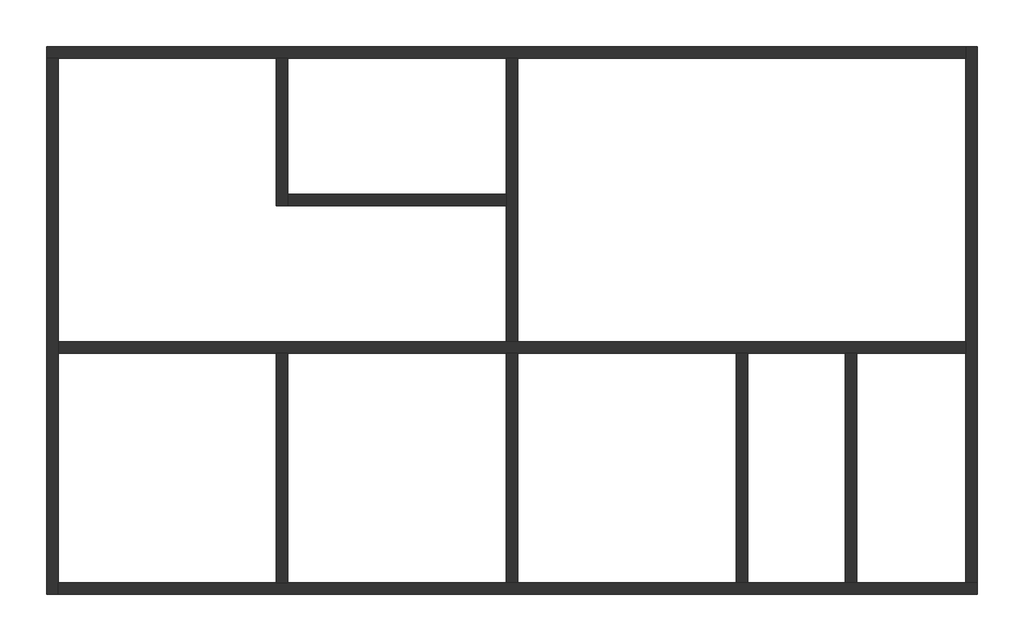
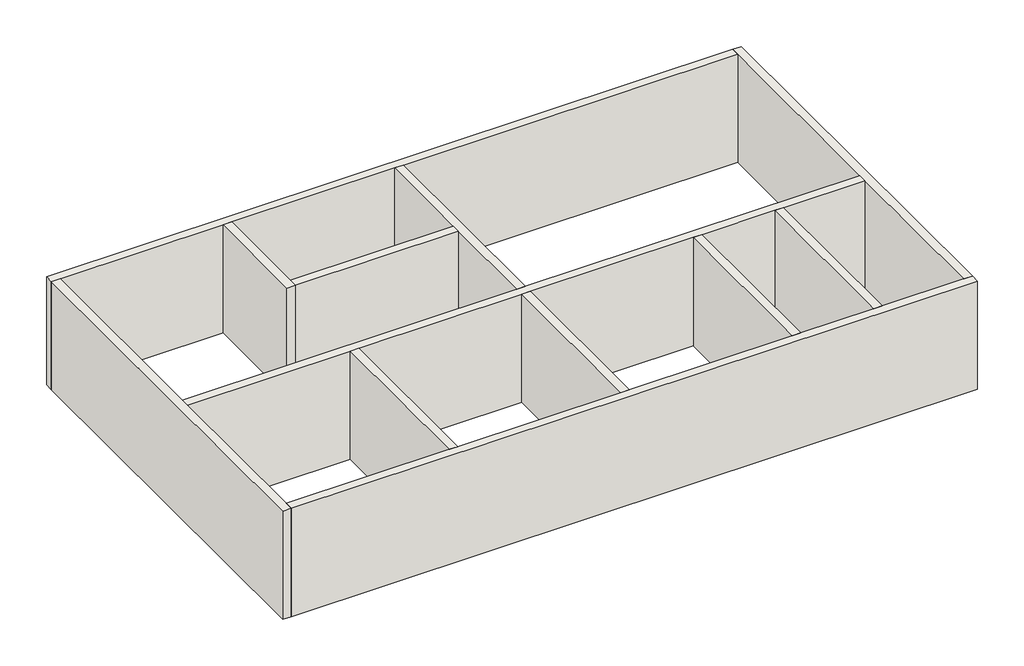
# One storey: 12 walls.
"""IFC4 building model written with IfcOpenShell, lengths in millimetres."""

from ifc_helpers import new_model, si_unit, frame, origin, place, context, project, spatial, polyline, outline, extrude, faceted_brep, element, save

model = new_model("IFC4")

# Units and contexts
model_context = context("Model", 3, world=origin())
ifc_project = project(units=[si_unit("LENGTHUNIT", "METRE", prefix="MILLI")], contexts=[model_context])

# Site, building, storey
site = spatial("IfcSite", under=ifc_project)
building = spatial("IfcBuilding", under=site)
storey = spatial("IfcBuildingStorey", under=building, Name="2nd FL GL+6,200", Elevation=6000.0)

# Walls
placement = place(None, origin())
element("IfcWall", 1, ObjectType="일반 - 300mm", at=placement, inside=storey, context=model_context, shape_type="Brep", body=[
    faceted_brep([(-18845.7273237, 9285.9763125, 6000.0), (-18545.7273237, 9285.9763125, 6000.0), (-12845.7273237, 9285.9763125, 6000.0), (-12545.7273237, 9285.9763125, 6000.0), (-6845.7273237, 9285.9763125, 6000.0), (-6545.7273237, 9285.9763125, 6000.0), (5154.2726763, 9285.9763125, 6000.0), (5154.2726763, 9285.9763125, 10000.0), (-6545.7273237, 9285.9763125, 10000.0), (-6845.7273237, 9285.9763125, 10000.0), (-12545.7273237, 9285.9763125, 10000.0), (-12845.7273237, 9285.9763125, 10000.0), (-18545.7273237, 9285.9763125, 10000.0), (-18845.7273237, 9285.9763125, 10000.0), (-18845.7273237, 9585.9763125, 6000.0), (-18845.7273237, 9585.9763125, 10000.0), (5154.2726763, 9585.9763125, 10000.0), (5154.2726763, 9585.9763125, 6000.0)], [[[0, 1, 2, 3, 4, 5, 6, 7, 8, 9, 10, 11, 12, 13]], [[14, 15, 16, 17]], [[6, 5, 4, 3, 2, 1, 0, 14, 17]], [[13, 12, 11, 10, 9, 8, 7, 16, 15]], [[0, 13, 15, 14]], [[7, 6, 17, 16]]]),
])
element("IfcWall", 2, ObjectType="일반 - 300mm", at=placement, inside=storey, context=model_context, shape_type="Brep", body=[
    faceted_brep([(-18545.7273237, -4714.0236875, 6000.0), (-18545.7273237, -4414.0236875, 6000.0), (-18545.7273237, 1585.9763125, 6000.0), (-18545.7273237, 1885.9763125, 6000.0), (-18545.7273237, 9285.9763125, 6000.0), (-18545.7273237, 9285.9763125, 10000.0), (-18545.7273237, 1885.9763125, 10000.0), (-18545.7273237, 1585.9763125, 10000.0), (-18545.7273237, -4414.0236875, 10000.0), (-18545.7273237, -4714.0236875, 10000.0), (-18845.7273237, -4714.0236875, 6000.0), (-18845.7273237, -4714.0236875, 10000.0), (-18845.7273237, 9285.9763125, 10000.0), (-18845.7273237, 9285.9763125, 6000.0)], [[[0, 1, 2, 3, 4, 5, 6, 7, 8, 9]], [[10, 11, 12, 13]], [[4, 3, 2, 1, 0, 10, 13]], [[9, 8, 7, 6, 5, 12, 11]], [[0, 9, 11, 10]], [[5, 4, 13, 12]]]),
])
element("IfcWall", 3, ObjectType="일반 - 300mm", at=placement, inside=storey, context=model_context, shape_type="Brep", body=[
    faceted_brep([(5454.2726763, -4414.0236875, 6000.0), (5154.2726763, -4414.0236875, 6000.0), (2304.2726763, -4414.0236875, 6000.0), (2004.2726763, -4414.0236875, 6000.0), (-545.7273237, -4414.0236875, 6000.0), (-845.7273237, -4414.0236875, 6000.0), (-6545.7273237, -4414.0236875, 6000.0), (-6845.7273237, -4414.0236875, 6000.0), (-12545.7273237, -4414.0236875, 6000.0), (-12845.7273237, -4414.0236875, 6000.0), (-18545.7273237, -4414.0236875, 6000.0), (-18545.7273237, -4414.0236875, 10000.0), (-12845.7273237, -4414.0236875, 10000.0), (-12545.7273237, -4414.0236875, 10000.0), (-6845.7273237, -4414.0236875, 10000.0), (-6545.7273237, -4414.0236875, 10000.0), (-845.7273237, -4414.0236875, 10000.0), (-545.7273237, -4414.0236875, 10000.0), (2004.2726763, -4414.0236875, 10000.0), (2304.2726763, -4414.0236875, 10000.0), (5154.2726763, -4414.0236875, 10000.0), (5454.2726763, -4414.0236875, 10000.0), (5454.2726763, -4714.0236875, 6000.0), (5454.2726763, -4714.0236875, 10000.0), (-18545.7273237, -4714.0236875, 10000.0), (-18545.7273237, -4714.0236875, 6000.0)], [[[0, 1, 2, 3, 4, 5, 6, 7, 8, 9, 10, 11, 12, 13, 14, 15, 16, 17, 18, 19, 20, 21]], [[22, 23, 24, 25]], [[10, 9, 8, 7, 6, 5, 4, 3, 2, 1, 0, 22, 25]], [[21, 20, 19, 18, 17, 16, 15, 14, 13, 12, 11, 24, 23]], [[0, 21, 23, 22]], [[11, 10, 25, 24]]]),
])
element("IfcWall", 4, ObjectType="일반 - 300mm", at=placement, inside=storey, context=model_context, shape_type="Brep", body=[
    faceted_brep([(5154.2726763, 9585.9763125, 6000.0), (5154.2726763, 9285.9763125, 6000.0), (5154.2726763, 1885.9763125, 6000.0), (5154.2726763, 1585.9763125, 6000.0), (5154.2726763, -4414.0236875, 6000.0), (5154.2726763, -4414.0236875, 10000.0), (5154.2726763, 1585.9763125, 10000.0), (5154.2726763, 1885.9763125, 10000.0), (5154.2726763, 9285.9763125, 10000.0), (5154.2726763, 9585.9763125, 10000.0), (5454.2726763, 9585.9763125, 6000.0), (5454.2726763, 9585.9763125, 10000.0), (5454.2726763, -4414.0236875, 10000.0), (5454.2726763, -4414.0236875, 6000.0)], [[[0, 1, 2, 3, 4, 5, 6, 7, 8, 9]], [[10, 11, 12, 13]], [[4, 3, 2, 1, 0, 10, 13]], [[9, 8, 7, 6, 5, 12, 11]], [[0, 9, 11, 10]], [[5, 4, 13, 12]]]),
])
element("IfcWall", 5, ObjectType="일반 - 300mm", at=placement, inside=storey, context=model_context, shape_type="Brep", body=[
    faceted_brep([(-12545.7273237, 5425.9613486, 6000.0), (-12545.7273237, 5725.9613486, 6000.0), (-12545.7273237, 9285.9763125, 6000.0), (-12545.7273237, 9285.9763125, 10000.0), (-12545.7273237, 5725.9613486, 10000.0), (-12545.7273237, 5425.9613486, 10000.0), (-12845.7273237, 5425.9613486, 6000.0), (-12845.7273237, 5425.9613486, 10000.0), (-12845.7273237, 9285.9763125, 10000.0), (-12845.7273237, 9285.9763125, 6000.0)], [[[0, 1, 2, 3, 4, 5]], [[6, 7, 8, 9]], [[2, 1, 0, 6, 9]], [[5, 4, 3, 8, 7]], [[3, 2, 9, 8]], [[0, 5, 7, 6]]]),
])
element("IfcWall", 6, ObjectType="일반 - 300mm", at=placement, inside=storey, context=model_context, shape_type="SweptSolid", body=[
    extrude(outline(polyline([(-6845.7273237, 5425.9613486), (-12545.7273237, 5425.9613486), (-12545.7273237, 5725.9613486), (-6845.7273237, 5725.9613486), (-6845.7273237, 5425.9613486)])), frame((0.0, 0.0, 6000.0), z_axis=(0.0, 0.0, 1.0), x_axis=(1.0, 0.0, 0.0)), (0.0, 0.0, 1.0), 4000.0),
])
element("IfcWall", 7, ObjectType="일반 - 300mm", at=placement, inside=storey, context=model_context, shape_type="Brep", body=[
    faceted_brep([(-6545.7273237, 1885.9763125, 6000.0), (-6545.7273237, 9285.9763125, 6000.0), (-6545.7273237, 9285.9763125, 10000.0), (-6545.7273237, 1885.9763125, 10000.0), (-6845.7273237, 1885.9763125, 6000.0), (-6845.7273237, 1885.9763125, 10000.0), (-6845.7273237, 5425.9613486, 10000.0), (-6845.7273237, 5725.9613486, 10000.0), (-6845.7273237, 9285.9763125, 10000.0), (-6845.7273237, 9285.9763125, 6000.0), (-6845.7273237, 5725.9613486, 6000.0), (-6845.7273237, 5425.9613486, 6000.0)], [[[0, 1, 2, 3]], [[4, 5, 6, 7, 8, 9, 10, 11]], [[1, 0, 4, 11, 10, 9]], [[3, 2, 8, 7, 6, 5]], [[2, 1, 9, 8]], [[0, 3, 5, 4]]]),
])
element("IfcWall", 8, ObjectType="일반 - 300mm", at=placement, inside=storey, context=model_context, shape_type="Brep", body=[
    faceted_brep([(-18545.7273237, 1585.9763125, 6000.0), (-12845.7273237, 1585.9763125, 6000.0), (-12545.7273237, 1585.9763125, 6000.0), (-6845.7273237, 1585.9763125, 6000.0), (-6545.7273237, 1585.9763125, 6000.0), (-845.7273237, 1585.9763125, 6000.0), (-545.7273237, 1585.9763125, 6000.0), (2004.2726763, 1585.9763125, 6000.0), (2304.2726763, 1585.9763125, 6000.0), (5154.2726763, 1585.9763125, 6000.0), (5154.2726763, 1585.9763125, 10000.0), (2304.2726763, 1585.9763125, 10000.0), (2004.2726763, 1585.9763125, 10000.0), (-545.7273237, 1585.9763125, 10000.0), (-845.7273237, 1585.9763125, 10000.0), (-6545.7273237, 1585.9763125, 10000.0), (-6845.7273237, 1585.9763125, 10000.0), (-12545.7273237, 1585.9763125, 10000.0), (-12845.7273237, 1585.9763125, 10000.0), (-18545.7273237, 1585.9763125, 10000.0), (-18545.7273237, 1885.9763125, 6000.0), (-18545.7273237, 1885.9763125, 10000.0), (-6845.7273237, 1885.9763125, 10000.0), (-6545.7273237, 1885.9763125, 10000.0), (5154.2726763, 1885.9763125, 10000.0), (5154.2726763, 1885.9763125, 6000.0), (-6545.7273237, 1885.9763125, 6000.0), (-6845.7273237, 1885.9763125, 6000.0)], [[[0, 1, 2, 3, 4, 5, 6, 7, 8, 9, 10, 11, 12, 13, 14, 15, 16, 17, 18, 19]], [[20, 21, 22, 23, 24, 25, 26, 27]], [[9, 8, 7, 6, 5, 4, 3, 2, 1, 0, 20, 27, 26, 25]], [[19, 18, 17, 16, 15, 14, 13, 12, 11, 10, 24, 23, 22, 21]], [[10, 9, 25, 24]], [[0, 19, 21, 20]]]),
])
element("IfcWall", 9, ObjectType="일반 - 300mm", at=placement, inside=storey, context=model_context, shape_type="SweptSolid", body=[
    extrude(outline(polyline([(2004.2726763, -4414.0236875), (2004.2726763, 1585.9763125), (2304.2726763, 1585.9763125), (2304.2726763, -4414.0236875), (2004.2726763, -4414.0236875)])), frame((0.0, 0.0, 6000.0), z_axis=(0.0, 0.0, 1.0), x_axis=(1.0, 0.0, 0.0)), (0.0, 0.0, 1.0), 4000.0),
])
element("IfcWall", 10, ObjectType="일반 - 300mm", at=placement, inside=storey, context=model_context, shape_type="SweptSolid", body=[
    extrude(outline(polyline([(-845.7273237, -4414.0236875), (-845.7273237, 1585.9763125), (-545.7273237, 1585.9763125), (-545.7273237, -4414.0236875), (-845.7273237, -4414.0236875)])), frame((0.0, 0.0, 6000.0), z_axis=(0.0, 0.0, 1.0), x_axis=(1.0, 0.0, 0.0)), (0.0, 0.0, 1.0), 4000.0),
])
element("IfcWall", 11, ObjectType="일반 - 300mm", at=placement, inside=storey, context=model_context, shape_type="SweptSolid", body=[
    extrude(outline(polyline([(-12845.7273237, -4414.0236875), (-12845.7273237, 1585.9763125), (-12545.7273237, 1585.9763125), (-12545.7273237, -4414.0236875), (-12845.7273237, -4414.0236875)])), frame((0.0, 0.0, 6000.0), z_axis=(0.0, 0.0, 1.0), x_axis=(1.0, 0.0, 0.0)), (0.0, 0.0, 1.0), 4000.0),
])
element("IfcWall", 12, ObjectType="일반 - 300mm", at=placement, inside=storey, context=model_context, shape_type="SweptSolid", body=[
    extrude(outline(polyline([(-6845.7273237, -4414.0236875), (-6845.7273237, 1585.9763125), (-6545.7273237, 1585.9763125), (-6545.7273237, -4414.0236875), (-6845.7273237, -4414.0236875)])), frame((0.0, 0.0, 6000.0), z_axis=(0.0, 0.0, 1.0), x_axis=(1.0, 0.0, 0.0)), (0.0, 0.0, 1.0), 4000.0),
])

save(model, "model.ifc")

# Revit data of these elements
# Type "일반 - 300mm"
#   Layers, outside or top first: 300 mm no material (function 1)
# Elements 1, 2, 3, 4, 5, 6, 7, 8, 9, 10, 11, 12 (IfcWall, "일반 - 300mm")
#   Comments = ""
#   Top Offset = 0 mm
#   Base Offset = 0 mm
#   Unconnected Height = 4000 mm
#   wall height = 4000 mm
#   Phase Created = 신축
#   Base Constraint = 2nd FL GL+6,200
#   Top Constraint = Roof GL+10,000
#   Materials on its faces: "기본 벽"
# Materials
#   "기본 벽": class "다양한", colour RGB 128 128 128, transparency 0, Cost = 0
# Room at (-9695.727, 7505.969) mm, phase "신축", upper level "2nd FL GL+6,200", upper offset 4000 mm, lower offset 0 mm
#   Base Finish = "B32"
#   Ceiling Finish = "C95A"
#   Wall Finish = "W32D"
#   Floor Finish = "F91"
#   Number = "2102"
#   Name = "test"
#   H_Room W = 0 mm
#   H_Room L = 0 mm
#   H_Room H or CH = 0 mm
# Room at (-15695.727, -1414.024) mm, phase "신축", upper level "2nd FL GL+6,200", upper offset 4000 mm, lower offset 0 mm
#   Base Finish = "B33"
#   Ceiling Finish = "C95A"
#   Wall Finish = "W01B"
#   Floor Finish = "F34B"
#   Number = "2108"
#   Name = "test"
#   H_Room W = 0 mm
#   H_Room L = 0 mm
#   H_Room H or CH = 0 mm
# Room at (-14870.067, 5585.976) mm, phase "신축", upper level "2nd FL GL+6,200", upper offset 4000 mm, lower offset 0 mm
#   Base Finish = "B03"
#   Ceiling Finish = "C01"
#   Wall Finish = "W04B"
#   Floor Finish = "F54A"
#   Number = "2101"
#   Name = "test"
#   H_Room W = 0 mm
#   H_Room L = 0 mm
#   H_Room H or CH = 0 mm
# Room at (-9695.727, -1414.024) mm, phase "신축", upper level "2nd FL GL+6,200", upper offset 4000 mm, lower offset 0 mm
#   Base Finish = "B32"
#   Ceiling Finish = "C01"
#   Wall Finish = "W01A"
#   Floor Finish = "F34A"
#   Number = "2107"
#   Name = "test"
#   H_Room W = 0 mm
#   H_Room L = 0 mm
#   H_Room H or CH = 0 mm
# Room at (-3695.727, -1414.024) mm, phase "신축", upper level "2nd FL GL+6,200", upper offset 4000 mm, lower offset 0 mm
#   Base Finish = "B03"
#   Ceiling Finish = "C96A"
#   Wall Finish = "W32D"
#   Floor Finish = "F31B"
#   Number = "2106"
#   Name = "test"
#   H_Room W = 0 mm
#   H_Room L = 0 mm
#   H_Room H or CH = 0 mm
# Room at (729.273, -1414.024) mm, phase "신축", upper level "2nd FL GL+6,200", upper offset 4000 mm, lower offset 0 mm
#   Base Finish = "B01"
#   Ceiling Finish = "C95A"
#   Wall Finish = "W04B"
#   Floor Finish = "F06A"
#   Number = "2105"
#   Name = "test"
#   H_Room W = 0 mm
#   H_Room L = 0 mm
#   H_Room H or CH = 0 mm
# Room at (-695.727, 5585.976) mm, phase "신축", upper level "2nd FL GL+6,200", upper offset 4000 mm, lower offset 0 mm
#   Base Finish = "B33"
#   Ceiling Finish = "C96A"
#   Wall Finish = "W01A"
#   Floor Finish = "F91"
#   Number = "2103"
#   Name = "test"
#   H_Room W = 0 mm
#   H_Room L = 0 mm
#   H_Room H or CH = 0 mm
# Room at (3729.273, -1414.024) mm, phase "신축", upper level "2nd FL GL+6,200", upper offset 4000 mm, lower offset 0 mm
#   Base Finish = "B35A"
#   Ceiling Finish = "C01"
#   Wall Finish = "W01B"
#   Floor Finish = "F03"
#   Number = "2104"
#   Name = "test"
#   H_Room W = 0 mm
#   H_Room L = 0 mm
#   H_Room H or CH = 0 mm
